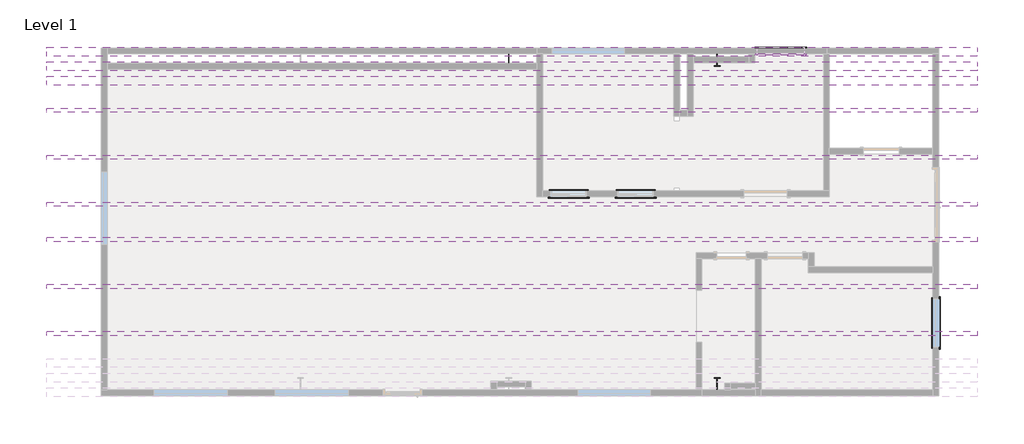
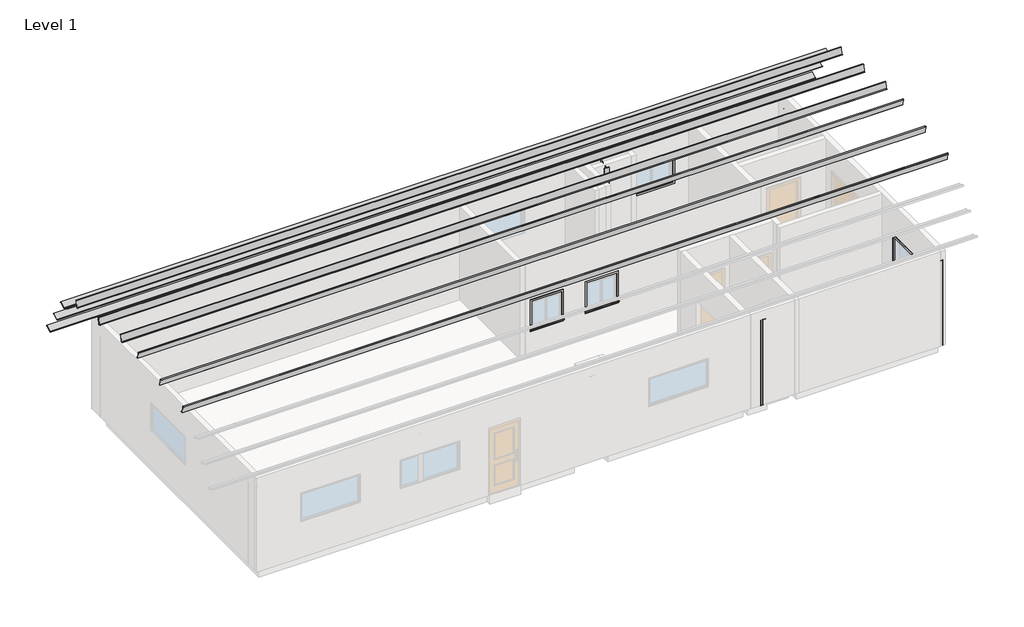
# One storey, part 3 of 3: 9 beams, 8 proxies, 5 columns.
"""IFC4 building model written with IfcOpenShell, lengths in millimetres."""

import ifcopenshell
import ifcopenshell.guid

model = None  # the IFC model being written
_history = None  # IfcOwnerHistory: only IFC2X3 demands one
_inside = {}  # id of a spatial element -> (the spatial element, [elements in it])
_under = {}  # id of a project, library or spatial element -> (it, [spatial elements below it])
_declared = {}  # id of a project -> (the project, [libraries it declares])
_typed = {}  # id of a type object -> (the type object, [elements of that type])
_made_of = {}  # id of a material, layer set ... -> (it, [elements and type objects made of it])


def new_model(schema):
    """Start an empty IFC model of exactly this schema.

    Asked for "IFC4X3", IfcOpenShell would pick the latest addendum, in which some entities
    have other attributes; the version numbers below select the first issue.
    IFC2X3 requires an IfcOwnerHistory on every rooted entity: one is made here for all.
    """
    global model, _history
    if schema == "IFC4X3":
        model = ifcopenshell.file(schema_version=(4, 3, 0, 0))
    else:
        model = ifcopenshell.file(schema=schema)
    _inside.clear()
    _under.clear()
    _declared.clear()
    _typed.clear()
    _made_of.clear()
    _history = None
    if model.schema == "IFC2X3":
        org = make("IfcOrganization", Name="unknown")
        user = make(
            "IfcPersonAndOrganization",
            ThePerson=make("IfcPerson", FamilyName="unknown"),
            TheOrganization=org,
        )
        app = make(
            "IfcApplication",
            ApplicationDeveloper=org,
            Version="unknown",
            ApplicationFullName="unknown",
            ApplicationIdentifier="unknown",
        )
        _history = make(
            "IfcOwnerHistory",
            OwningUser=user,
            OwningApplication=app,
            ChangeAction="ADDED",
            CreationDate=0,
        )
    return model


def make(cls, **values):
    """One entity of the class cls with the attributes given. An attribute that is None is left unset."""
    return model.create_entity(
        cls, **{name: value for name, value in values.items() if value is not None}
    )


def rooted(cls, **values):
    """An entity with a GlobalId (a new one), such as an element, a storey or a relation."""
    return make(cls, GlobalId=ifcopenshell.guid.new(), OwnerHistory=_history, **values)


def si_unit(unit_type, name, prefix=None):
    """IfcSIUnit, for example si_unit("LENGTHUNIT", "METRE", prefix="MILLI")."""
    return make("IfcSIUnit", UnitType=unit_type, Prefix=prefix, Name=name)


def assignment(units):
    """IfcUnitAssignment: the units of a project."""
    return None if units is None else make("IfcUnitAssignment", Units=units)


def point(xyz):
    """IfcCartesianPoint."""
    return None if xyz is None else make("IfcCartesianPoint", Coordinates=xyz)


def direction(xyz):
    """IfcDirection."""
    return None if xyz is None else make("IfcDirection", DirectionRatios=xyz)


def frame(location, z_axis=None, x_axis=None):
    """IfcAxis2Placement3D, a coordinate frame: its origin and axes. An axis left out is left unset."""
    return make(
        "IfcAxis2Placement3D",
        Location=point(location),
        Axis=direction(z_axis),
        RefDirection=direction(x_axis),
    )


def origin():
    """The frame at (0, 0, 0) with its axes left unset."""
    return frame((0.0, 0.0, 0.0))


def origin_with_axes():
    """The frame at (0, 0, 0) with the z axis (0, 0, 1) and the x axis (1, 0, 0) written out."""
    return frame((0.0, 0.0, 0.0), z_axis=(0.0, 0.0, 1.0), x_axis=(1.0, 0.0, 0.0))


def place(relative_to, where):
    """IfcLocalPlacement: puts the frame where relative to a parent placement (None: the world)."""
    return make(
        "IfcLocalPlacement", PlacementRelTo=relative_to, RelativePlacement=where
    )


def context(
    kind, dimensions, precision=None, world=None, true_north=None, identifier=None
):
    """IfcGeometricRepresentationContext, for example the 3D "Model" context."""
    return make(
        "IfcGeometricRepresentationContext",
        ContextIdentifier=identifier,
        ContextType=kind,
        CoordinateSpaceDimension=dimensions,
        Precision=precision,
        WorldCoordinateSystem=world,
        TrueNorth=true_north,
    )


def project(units=None, contexts=None):
    """IfcProject with its units and contexts."""
    return rooted(
        "IfcProject",
        Name="project",
        RepresentationContexts=contexts,
        UnitsInContext=assignment(units),
    )


def spatial(cls, under=None, at=None, **own):
    """A site, building, storey or space (cls), placed at a placement, below another one or the project."""
    s = rooted(cls, ObjectPlacement=at, **own)
    if under is not None:
        _under.setdefault(under.id(), (under, []))[1].append(s)
    return s


def polyline(points):
    """IfcPolyline through the points."""
    return make("IfcPolyline", Points=[point(p) for p in points])


def circle_curve(where, radius):
    """IfcCircle in the frame where."""
    return make("IfcCircle", Position=where, Radius=radius)


def ellipse_curve(where, semi_axis1, semi_axis2):
    """IfcEllipse in the frame where."""
    return make(
        "IfcEllipse", Position=where, SemiAxis1=semi_axis1, SemiAxis2=semi_axis2
    )


def outline(outer, holes=None, kind="AREA"):
    """IfcArbitraryClosedProfileDef: a profile drawn as a closed curve; with holes, ...WithVoids."""
    if holes is None:
        return make("IfcArbitraryClosedProfileDef", ProfileType=kind, OuterCurve=outer)
    return make(
        "IfcArbitraryProfileDefWithVoids",
        ProfileType=kind,
        OuterCurve=outer,
        InnerCurves=holes,
    )


def extrude(swept, where, along, depth):
    """IfcExtrudedAreaSolid: the profile swept, set in the frame where, extruded along a direction by depth."""
    return make(
        "IfcExtrudedAreaSolid",
        SweptArea=swept,
        Position=where,
        ExtrudedDirection=direction(along),
        Depth=depth,
    )


def shape(context_of_items, identifier, shape_type, items):
    """IfcShapeRepresentation: the items that make up one representation, for example the "Body"."""
    return make(
        "IfcShapeRepresentation",
        ContextOfItems=context_of_items,
        RepresentationIdentifier=identifier,
        RepresentationType=shape_type,
        Items=items,
    )


def source(mapping_origin, context_of_items, identifier, shape_type, items):
    """IfcRepresentationMap: a shape defined once, which mapped items show again and again."""
    return make(
        "IfcRepresentationMap",
        MappingOrigin=mapping_origin,
        MappedRepresentation=shape(context_of_items, identifier, shape_type, items),
    )


def transform(
    local_origin,
    x_axis=None,
    y_axis=None,
    z_axis=None,
    scale=None,
    scale2=None,
    scale3=None,
    uniform=True,
):
    """IfcCartesianTransformationOperator3D, or its non-uniform kind. x_axis, y_axis, z_axis: its Axis1, 2, 3."""
    if uniform:
        return make(
            "IfcCartesianTransformationOperator3D",
            Axis1=direction(x_axis),
            Axis2=direction(y_axis),
            LocalOrigin=point(local_origin),
            Scale=scale,
            Axis3=direction(z_axis),
        )
    return make(
        "IfcCartesianTransformationOperator3DnonUniform",
        Axis1=direction(x_axis),
        Axis2=direction(y_axis),
        LocalOrigin=point(local_origin),
        Scale=scale,
        Axis3=direction(z_axis),
        Scale2=scale2,
        Scale3=scale3,
    )


def mapped(mapping_source, mapping_target):
    """IfcMappedItem: shows the shape of a source again, moved by a transform."""
    return make(
        "IfcMappedItem", MappingSource=mapping_source, MappingTarget=mapping_target
    )


def made_of(thing, what):
    """Note that an element or type object is made of a material, layer set ...; save() writes the relation."""
    if what is not None:
        _made_of.setdefault(what.id(), (what, []))[1].append(thing)
    return thing


def element(
    cls,
    number,
    at=None,
    inside=None,
    cuts=None,
    type_object=None,
    material=None,
    context=None,
    identifier="Body",
    shape_type=None,
    held_by="IfcProductDefinitionShape",
    body=None,
    shapes=None,
    **own,
):
    """One element of the class cls, such as IfcWall. Its Tag is "e" and its number.

    at: its placement. inside: the storey or other place that contains it. cuts: it is an
    opening in that element (IfcRelVoidsElement). A single representation is given by context,
    identifier, shape_type and body (its items); several are given by shapes. held_by: the class
    of the entity that holds the representations. save() writes the other relations.
    """
    e = rooted(cls, Tag="e%d" % number, ObjectPlacement=at, **own)
    if body is not None:
        shapes = [shape(context, identifier, shape_type, body)]
    if shapes is not None:
        e.Representation = make(held_by, Representations=shapes)
    if inside is not None:
        _inside.setdefault(inside.id(), (inside, []))[1].append(e)
    if cuts is not None:
        rooted(
            "IfcRelVoidsElement", RelatingBuildingElement=cuts, RelatedOpeningElement=e
        )
    if type_object is not None:
        _typed.setdefault(type_object.id(), (type_object, []))[1].append(e)
    return made_of(e, material)


def aggregate(whole, parts):
    """IfcRelAggregates: a whole, such as a stair, and the parts it consists of."""
    return rooted("IfcRelAggregates", RelatingObject=whole, RelatedObjects=parts)


def save(model, path):
    """Write the relations noted so far, then the file.

    IfcRelAggregates (storeys below a building ...), IfcRelContainedInSpatialStructure (elements
    in a storey), IfcRelDefinesByType, IfcRelAssociatesMaterial and IfcRelDeclares: one each for
    every whole, place, type object, material and project.
    """
    for whole, parts in _under.values():
        aggregate(whole, parts)
    for where, things in _inside.values():
        rooted(
            "IfcRelContainedInSpatialStructure",
            RelatedElements=things,
            RelatingStructure=where,
        )
    for kind, things in _typed.values():
        rooted("IfcRelDefinesByType", RelatedObjects=things, RelatingType=kind)
    for what, things in _made_of.values():
        rooted("IfcRelAssociatesMaterial", RelatedObjects=things, RelatingMaterial=what)
    for by, libraries in _declared.values():
        rooted("IfcRelDeclares", RelatingContext=by, RelatedDefinitions=libraries)
    model.write(path)


def plane_surface(at):
    """IfcPlane: the flat surface through the origin of the frame at, square to its z axis."""
    return make("IfcPlane", Position=at)


def revolved_surface(curve, axis_point, axis_direction):
    """IfcSurfaceOfRevolution: the curve turned about the line through axis_point along axis_direction."""
    return make(
        "IfcSurfaceOfRevolution",
        SweptCurve=make("IfcArbitraryOpenProfileDef", ProfileType="CURVE", Curve=curve),
        AxisPosition=make("IfcAxis1Placement", Location=point(axis_point), Axis=direction(axis_direction)),
    )


def advanced_brep(points, edges, surfaces, faces):
    """IfcAdvancedBrep: a solid bounded by faces that lie on surfaces and meet in shared edges.

    An edge is (start, end): straight between two places in points (the first is 0);
    or (start, end, curve); or (start, end, curve, False) where it runs against its curve.
    A face is (place in surfaces, loops), or (place, loops, False) where it looks against
    its surface's normal. A loop lists edges by number (the first is 1), with a minus sign
    where the edge is run from its end to its start. The first loop is the outer one.
    """
    corners = [point(p) for p in points]
    vertices = [make("IfcVertexPoint", VertexGeometry=c) for c in corners]
    made = []
    for start, end, *more in edges:
        made.append(
            make(
                "IfcEdgeCurve",
                EdgeStart=vertices[start],
                EdgeEnd=vertices[end],
                EdgeGeometry=more[0] if more else make("IfcPolyline", Points=[corners[start], corners[end]]),
                SameSense=more[1] if len(more) > 1 else True,
            )
        )
    hull = []
    for where, loops, *sense in faces:
        bounds = []
        for j, loop in enumerate(loops):
            ring = [make("IfcOrientedEdge", EdgeElement=made[abs(k) - 1], Orientation=k > 0) for k in loop]
            bounds.append(
                make(
                    "IfcFaceOuterBound" if j == 0 else "IfcFaceBound",
                    Bound=make("IfcEdgeLoop", EdgeList=ring),
                    Orientation=True,
                )
            )
        hull.append(make("IfcAdvancedFace", Bounds=bounds, FaceSurface=surfaces[where], SameSense=sense[0] if sense else True))
    return make("IfcAdvancedBrep", Outer=make("IfcClosedShell", CfsFaces=hull))


def z_shapes_z_3x8_0ff4bf34(model_context):
    return source(origin(), model_context, "Body", "SweptSolid", [
        extrude(outline(polyline([(-57.2805719, 101.596825), (-57.2805719, 111.248825), (-19.1805719, 111.248825), (-19.1805719, -101.603175), (18.9194281, -101.603175), (18.9194281, -107.953175), (-27.1991352, -107.953175), (-27.1991352, 101.596825), (-57.2805719, 101.596825)])), frame((-11963.4, 0.0, 0.0), z_axis=(1.0, 0.0, 0.0), x_axis=(0.0, 1.0, 0.0)), (0.0, 0.0, 1.0), 23926.8),
    ])


def trim_window_exterior_flat_with_sill_c4e67c73(model_context):
    return source(origin(), model_context, "Body", "SweptSolid", [
        extrude(outline(polyline([(666.75, -936.5823709), (666.75, -993.7323709), (-666.75, -993.7323709), (-666.75, -936.5823709), (666.75, -936.5823709)])), origin_with_axes(), (0.0, 0.0, 1.0), 19.05),
        extrude(outline(polyline([(-946.15, 38.1), (-916.8580645, 38.1), (-914.4, 19.05), (-914.4, 0.0), (-936.5823709, 0.0), (-936.5823709, 19.05), (-946.15, 19.05), (-946.15, 38.1)])), frame((-679.45, 0.0, 0.0), z_axis=(1.0, 0.0, 0.0), x_axis=(0.0, 1.0, 0.0)), (0.0, 0.0, 1.0), 1358.9),
        extrude(outline(polyline([(-666.75, 57.15), (666.75, 57.15), (666.75, -914.4), (609.6, -914.4), (609.6, 0.0), (-609.6, 0.0), (-609.6, -914.4), (-666.75, -914.4), (-666.75, 57.15)])), origin_with_axes(), (0.0, 0.0, 1.0), 19.05),
    ])


def trim_window_exterior_flat_with_sill_84e24481(model_context):
    return source(origin(), model_context, "Body", "SweptSolid", [
        extrude(outline(polyline([(514.35, -936.5823709), (514.35, -993.7323709), (-514.35, -993.7323709), (-514.35, -936.5823709), (514.35, -936.5823709)])), origin_with_axes(), (0.0, 0.0, 1.0), 19.05),
        extrude(outline(polyline([(-946.15, 38.1), (-916.8580645, 38.1), (-914.4, 19.05), (-914.4, 0.0), (-936.5823709, 0.0), (-936.5823709, 19.05), (-946.15, 19.05), (-946.15, 38.1)])), frame((-527.05, 0.0, 0.0), z_axis=(1.0, 0.0, 0.0), x_axis=(0.0, 1.0, 0.0)), (0.0, 0.0, 1.0), 1054.1),
        extrude(outline(polyline([(-514.35, 57.15), (514.35, 57.15), (514.35, -914.4), (457.2, -914.4), (457.2, 0.0), (-457.2, 0.0), (-457.2, -914.4), (-514.35, -914.4), (-514.35, 57.15)])), origin_with_axes(), (0.0, 0.0, 1.0), 19.05),
    ])


def trim_window_interior_flat_picture_frame_cf1733af(model_context):
    return source(origin(), model_context, "Body", "SweptSolid", [
        extrude(outline(polyline([(654.05, 44.45), (654.05, -958.85), (-654.05, -958.85), (-654.05, 44.45), (654.05, 44.45)]), holes=[polyline([(596.9, -12.7), (-596.9, -12.7), (-596.9, -901.7), (596.9, -901.7), (596.9, -12.7)])]), origin_with_axes(), (0.0, 0.0, 1.0), 31.75),
    ])


def trim_window_interior_flat_picture_frame_28d4e5dc(model_context):
    return source(origin(), model_context, "Body", "SweptSolid", [
        extrude(outline(polyline([(501.65, 44.45), (501.65, -958.85), (-501.65, -958.85), (-501.65, 44.45), (501.65, 44.45)]), holes=[polyline([(444.5, -12.7), (-444.5, -12.7), (-444.5, -901.7), (444.5, -901.7), (444.5, -12.7)])]), origin_with_axes(), (0.0, 0.0, 1.0), 31.75),
    ])


model = new_model("IFC4")

# Units and contexts
model_context = context("Model", 3, world=origin())
ifc_project = project(units=[si_unit("LENGTHUNIT", "METRE", prefix="MILLI")], contexts=[model_context])

# Site, building, storey
site = spatial("IfcSite", under=ifc_project)
building = spatial("IfcBuilding", under=site)
storey = spatial("IfcBuildingStorey", under=building, Name="Level 1", Elevation=0.0)

# Beams
placement = place(None, origin())
z_shapes_z_3x8_shape = z_shapes_z_3x8_0ff4bf34(model_context)
element("IfcBeam", 1, ObjectType="Z Shapes : Z 3X8", at=placement, inside=storey, context=model_context, shape_type="MappedRepresentation", body=[
    mapped(z_shapes_z_3x8_shape, transform((18060.1870052, 9961.4548323, 4912.1209483), x_axis=(-1.0, 0.0, 0.0), y_axis=(0.0, -0.9907950027882196, 0.13537083308413195), z_axis=(0.0, 0.13537083308413195, 0.9907950027882196))),
])
element("IfcBeam", 2, ObjectType="Z Shapes : Z 3X8", at=placement, inside=storey, context=model_context, shape_type="MappedRepresentation", body=[
    mapped(z_shapes_z_3x8_shape, transform((18060.1870052, 8753.4775649, 5077.165068), x_axis=(-1.0, 0.0, 0.0), y_axis=(0.0, -0.9907950027882196, 0.13537083308413195), z_axis=(0.0, 0.13537083308413195, 0.9907950027882196))),
])
element("IfcBeam", 3, ObjectType="Z Shapes : Z 3X8", at=placement, inside=storey, context=model_context, shape_type="MappedRepresentation", body=[
    mapped(z_shapes_z_3x8_shape, transform((18060.1870052, 7545.5002975, 5242.2091877), x_axis=(-1.0, 0.0, 0.0), y_axis=(0.0, -0.9907950027882196, 0.13537083308413195), z_axis=(0.0, 0.13537083308413195, 0.9907950027882196))),
])
element("IfcBeam", 4, ObjectType="Z Shapes : Z 3X8", at=placement, inside=storey, context=model_context, shape_type="MappedRepresentation", body=[
    mapped(z_shapes_z_3x8_shape, transform((18060.1870052, 6681.0227757, 5242.2091877), x_axis=(1.0, 0.0, 0.0), y_axis=(0.0, 0.9907950027882196, 0.13537083308413195), z_axis=(0.0, -0.13537083308413195, 0.9907950027882196))),
])
element("IfcBeam", 5, ObjectType="Z Shapes : Z 3X8", at=placement, inside=storey, context=model_context, shape_type="MappedRepresentation", body=[
    mapped(z_shapes_z_3x8_shape, transform((18060.1870052, 5473.0455083, 5077.165068), x_axis=(1.0, 0.0, 0.0), y_axis=(0.0, 0.9907950027882196, 0.13537083308413195), z_axis=(0.0, -0.13537083308413195, 0.9907950027882196))),
])
element("IfcBeam", 6, ObjectType="Z Shapes : Z 3X8", at=placement, inside=storey, context=model_context, shape_type="MappedRepresentation", body=[
    mapped(z_shapes_z_3x8_shape, transform((18060.1870052, 4265.0682409, 4912.1209483), x_axis=(1.0, 0.0, 0.0), y_axis=(0.0, 0.9907950027882196, 0.13537083308413195), z_axis=(0.0, -0.13537083308413195, 0.9907950027882196))),
])
element("IfcBeam", 7, ObjectType="Z Shapes : Z 3X8", at=placement, inside=storey, context=model_context, shape_type="MappedRepresentation", body=[
    mapped(z_shapes_z_3x8_shape, transform((18060.1870052, 10729.7081219, 4436.794501), x_axis=(-1.0, 0.0, 0.0), y_axis=(0.0, -0.5198738321222813, 0.8542430559708952), z_axis=(0.0, 0.8542430559708952, 0.5198738321222813))),
])
element("IfcBeam", 8, ObjectType="Z Shapes : Z 3X8", at=placement, inside=storey, context=model_context, shape_type="MappedRepresentation", body=[
    mapped(z_shapes_z_3x8_shape, transform((18060.1870052, 11104.2691119, 3821.3256987), x_axis=(-1.0, 0.0, 0.0), y_axis=(0.0, -0.5198738321222813, 0.8542430559708952), z_axis=(0.0, 0.8542430559708952, 0.5198738321222813))),
])
element("IfcBeam", 9, ObjectType="Z Shapes : Z 3X8", at=placement, inside=storey, context=model_context, shape_type="MappedRepresentation", body=[
    mapped(z_shapes_z_3x8_shape, transform((18060.1870052, 11478.830102, 3205.8568965), x_axis=(-1.0, 0.0, 0.0), y_axis=(0.0, -0.5198738321222813, 0.8542430559708952), z_axis=(0.0, 0.8542430559708952, 0.5198738321222813))),
])

# Proxies
trim_window_exterior_flat_with_sill_shape = trim_window_exterior_flat_with_sill_c4e67c73(model_context)
element("IfcBuildingElementProxy", 10, Name="Trim-Window-Exterior-Flat : with Sill", ObjectType="Trim-Window-Exterior-Flat : with Sill", at=placement, inside=storey, context=model_context, shape_type="MappedRepresentation", body=[
    mapped(trim_window_exterior_flat_with_sill_shape, transform((24967.1591867, 11583.6615366, 2166.9735008), x_axis=(-1.0, 0.0, 0.0), y_axis=(0.0, 0.0, 1.0), z_axis=(0.0, 1.0, 0.0))),
])
element("IfcBuildingElementProxy", 11, Name="Trim-Window-Exterior-Flat : with Sill", ObjectType="Trim-Window-Exterior-Flat : with Sill", at=placement, inside=storey, context=model_context, shape_type="MappedRepresentation", body=[
    mapped(trim_window_exterior_flat_with_sill_shape, transform((29032.9870052, 4516.1115366, 2108.2), x_axis=(0.0, 1.0, 0.0), y_axis=(0.0, 0.0, 1.0), z_axis=(1.0, 0.0, 0.0))),
])
trim_window_exterior_flat_with_sill_2_shape = trim_window_exterior_flat_with_sill_84e24481(model_context)
element("IfcBuildingElementProxy", 12, Name="Trim-Window-Exterior-Flat : with Sill", ObjectType="Trim-Window-Exterior-Flat : with Sill", at=placement, inside=storey, context=model_context, shape_type="MappedRepresentation", body=[
    mapped(trim_window_exterior_flat_with_sill_2_shape, transform((19514.3370052, 7760.9615366, 1828.8), x_axis=(1.0, 0.0, 0.0), y_axis=(0.0, 0.0, 1.0), z_axis=(0.0, -1.0, 0.0))),
])
element("IfcBuildingElementProxy", 13, Name="Trim-Window-Exterior-Flat : with Sill", ObjectType="Trim-Window-Exterior-Flat : with Sill", at=placement, inside=storey, context=model_context, shape_type="MappedRepresentation", body=[
    mapped(trim_window_exterior_flat_with_sill_2_shape, transform((21235.1870052, 7760.9615366, 1828.8), x_axis=(1.0, 0.0, 0.0), y_axis=(0.0, 0.0, 1.0), z_axis=(0.0, -1.0, 0.0))),
])
trim_window_interior_flat_picture_frame_shape = trim_window_interior_flat_picture_frame_cf1733af(model_context)
element("IfcBuildingElementProxy", 14, Name="Trim-Window-Interior-Flat : Picture Frame", ObjectType="Trim-Window-Interior-Flat : Picture Frame", at=placement, inside=storey, context=model_context, shape_type="MappedRepresentation", body=[
    mapped(trim_window_interior_flat_picture_frame_shape, transform((24967.1591867, 11431.2615366, 2166.9735008), x_axis=(1.0, 0.0, 0.0), y_axis=(0.0, 0.0, 1.0), z_axis=(0.0, -1.0, 0.0))),
])
element("IfcBuildingElementProxy", 15, Name="Trim-Window-Interior-Flat : Picture Frame", ObjectType="Trim-Window-Interior-Flat : Picture Frame", at=placement, inside=storey, context=model_context, shape_type="MappedRepresentation", body=[
    mapped(trim_window_interior_flat_picture_frame_shape, transform((28880.5870052, 4516.1115366, 2108.2), x_axis=(0.0, -1.0, 0.0), y_axis=(0.0, 0.0, 1.0), z_axis=(-1.0, 0.0, 0.0))),
])
trim_window_interior_flat_picture_frame_2_shape = trim_window_interior_flat_picture_frame_28d4e5dc(model_context)
element("IfcBuildingElementProxy", 16, Name="Trim-Window-Interior-Flat : Picture Frame", ObjectType="Trim-Window-Interior-Flat : Picture Frame", at=placement, inside=storey, context=model_context, shape_type="MappedRepresentation", body=[
    mapped(trim_window_interior_flat_picture_frame_2_shape, transform((19514.3370052, 7913.3615366, 1828.8), x_axis=(-1.0, 0.0, 0.0), y_axis=(0.0, 0.0, 1.0), z_axis=(0.0, 1.0, 0.0))),
])
element("IfcBuildingElementProxy", 17, Name="Trim-Window-Interior-Flat : Picture Frame", ObjectType="Trim-Window-Interior-Flat : Picture Frame", at=placement, inside=storey, context=model_context, shape_type="MappedRepresentation", body=[
    mapped(trim_window_interior_flat_picture_frame_2_shape, transform((21235.1870052, 7913.3615366, 1828.8), x_axis=(-1.0, 0.0, 0.0), y_axis=(0.0, 0.0, 1.0), z_axis=(0.0, 1.0, 0.0))),
])

# Columns
element("IfcColumn", 18, ObjectType="W-Wide Flange-Column : W6X18.5", at=placement, inside=storey, context=model_context, shape_type="AdvancedBrep", body=[
    advanced_brep(
    [(29032.9870052, 11583.6615366, 0.0), (29032.9870052, 11573.3745366, 0.0), (28972.0270052, 11573.3745366, 0.0), (28960.0890052, 11561.4365366, 0.0), (28960.0890052, 11135.9865366, 0.0), (28972.0270052, 11124.0485366, 0.0), (29032.9870052, 11124.0485366, 0.0), (29032.9870052, 11113.7615366, 0.0), (28880.5870052, 11113.7615366, 0.0), (28880.5870052, 11124.0485366, 0.0), (28941.5470052, 11124.0485366, 0.0), (28953.4850052, 11135.9865366, 0.0), (28953.4850052, 11561.4365366, 0.0), (28941.5470052, 11573.3745366, 0.0), (28880.5870052, 11573.3745366, 0.0), (28880.5870052, 11583.6615366, 0.0), (29032.9870052, 11583.6615366, 2825.947988), (29032.9870052, 11573.3745366, 2823.0639572), (28972.0270052, 11573.3745366, 2823.0639572), (28960.0890052, 11561.4365366, 2819.7170571), (28960.0890052, 11135.9865366, 2700.4392375), (28972.0270052, 11124.0485366, 2697.0923375), (29032.9870052, 11124.0485366, 2697.0923375), (29032.9870052, 11113.7615366, 2694.2083066), (28880.5870052, 11113.7615366, 2694.2083066), (28880.5870052, 11124.0485366, 2697.0923375), (28941.5470052, 11124.0485366, 2697.0923375), (28953.4850052, 11135.9865366, 2700.4392375), (28953.4850052, 11561.4365366, 2819.7170571), (28941.5470052, 11573.3745366, 2823.0639572), (28880.5870052, 11573.3745366, 2823.0639572), (28880.5870052, 11583.6615366, 2825.947988)],
    [
        (0, 1),
        (1, 2),
        (2, 3, circle_curve(frame((28972.0270052, 11561.4365366, 0.0), z_axis=(0.0, 0.0, 1.0), x_axis=(1.0, 0.0, 0.0)), 11.938)),
        (3, 4),
        (4, 5, circle_curve(frame((28972.0270052, 11135.9865366, 0.0), z_axis=(0.0, 0.0, 1.0), x_axis=(1.0, 0.0, 0.0)), 11.938)),
        (5, 6),
        (6, 7),
        (7, 8),
        (8, 9),
        (9, 10),
        (10, 11, circle_curve(frame((28941.5470052, 11135.9865366, 0.0), z_axis=(0.0, 0.0, 1.0), x_axis=(1.0, 0.0, 0.0)), 11.938)),
        (11, 12),
        (12, 13, circle_curve(frame((28941.5470052, 11561.4365366, 0.0), z_axis=(0.0, 0.0, 1.0), x_axis=(1.0, 0.0, 0.0)), 11.938)),
        (13, 14),
        (14, 15),
        (15, 0),
        (0, 16),
        (16, 17),
        (17, 1),
        (17, 18),
        (18, 2),
        (18, 19, ellipse_curve(frame((28972.0270052, 11561.4365366, 2819.7170571), z_axis=(0.0, -0.2699485280248176, 0.9628747541696346), x_axis=(0.0, -0.9628747541696346, -0.2699485280248172)), 12.3982895, 11.938)),
        (19, 3),
        (19, 20),
        (20, 4),
        (20, 21, ellipse_curve(frame((28972.0270052, 11135.9865366, 2700.4392375), z_axis=(0.0, -0.2699485280248176, 0.9628747541696346), x_axis=(0.0, -0.9628747541696346, -0.2699485280248172)), 12.3982895, 11.938)),
        (21, 5),
        (21, 22),
        (22, 6),
        (22, 23),
        (23, 7),
        (23, 24),
        (24, 8),
        (24, 25),
        (25, 9),
        (25, 26),
        (26, 10),
        (26, 27, ellipse_curve(frame((28941.5470052, 11135.9865366, 2700.4392375), z_axis=(0.0, -0.2699485280248176, 0.9628747541696346), x_axis=(0.0, -0.9628747541696346, -0.2699485280248172)), 12.3982895, 11.938)),
        (27, 11),
        (27, 28),
        (28, 12),
        (28, 29, ellipse_curve(frame((28941.5470052, 11561.4365366, 2819.7170571), z_axis=(0.0, -0.2699485280248176, 0.9628747541696346), x_axis=(0.0, -0.9628747541696346, -0.2699485280248172)), 12.3982895, 11.938)),
        (29, 13),
        (29, 30),
        (30, 14),
        (30, 31),
        (31, 15),
        (31, 16),
    ],
    [
        plane_surface(frame((28880.5870052, 11583.6615366, 0.0), z_axis=(0.0, 0.0, -1.0), x_axis=(1.0, 0.0, 0.0))),
        plane_surface(frame((29032.9870052, 11573.3745366, 2832.1), z_axis=(1.0, 0.0, 0.0), x_axis=(0.0, 0.0, -1.0))),
        plane_surface(frame((28972.0270052, 11573.3745366, 2832.1), z_axis=(0.0, -1.0, 0.0), x_axis=(0.0, 0.0, -1.0))),
        revolved_surface(polyline([(28983.9650052, 11561.4365366, 0.0), (28983.9650052, 11561.4365366, 2823.0639572)]), (28972.0270052, 11561.4365366, 0.0), (0.0, 0.0, -1.0)),
        plane_surface(frame((28960.0890052, 11135.9865366, 2832.1), z_axis=(1.0, 0.0, 0.0), x_axis=(0.0, 0.0, -1.0))),
        revolved_surface(polyline([(28983.9650052, 11135.9865366, 0.0), (28983.9650052, 11135.9865366, 2703.786137500551)]), (28972.0270052, 11135.9865366, 0.0), (0.0, 0.0, -1.0)),
        plane_surface(frame((29032.9870052, 11124.0485366, 2832.1), z_axis=(0.0, 1.0, 0.0), x_axis=(0.0, 0.0, -1.0))),
        plane_surface(frame((29032.9870052, 11113.7615366, 2832.1), z_axis=(1.0, 0.0, 0.0), x_axis=(0.0, 0.0, -1.0))),
        plane_surface(frame((28880.5870052, 11113.7615366, 2832.1), z_axis=(0.0, -1.0, 0.0), x_axis=(0.0, 0.0, -1.0))),
        plane_surface(frame((28880.5870052, 11124.0485366, 2832.1), z_axis=(-1.0, 0.0, 0.0), x_axis=(0.0, 0.0, -1.0))),
        plane_surface(frame((28941.5470052, 11124.0485366, 2832.1), z_axis=(0.0, 1.0, 0.0), x_axis=(0.0, 0.0, -1.0))),
        revolved_surface(polyline([(28953.485005199997, 11135.9865366, 0.0), (28953.485005199997, 11135.9865366, 2703.786137500551)]), (28941.5470052, 11135.9865366, 0.0), (0.0, 0.0, -1.0)),
        plane_surface(frame((28953.4850052, 11561.4365366, 2832.1), z_axis=(-1.0, 0.0, 0.0), x_axis=(0.0, 0.0, -1.0))),
        revolved_surface(polyline([(28953.485005199997, 11561.4365366, 0.0), (28953.485005199997, 11561.4365366, 2823.0639572)]), (28941.5470052, 11561.4365366, 0.0), (0.0, 0.0, -1.0)),
        plane_surface(frame((28880.5870052, 11573.3745366, 2832.1), z_axis=(0.0, -1.0, 0.0), x_axis=(0.0, 0.0, -1.0))),
        plane_surface(frame((28880.5870052, 11583.6615366, 2832.1), z_axis=(-1.0, 0.0, 0.0), x_axis=(0.0, 0.0, -1.0))),
        plane_surface(frame((29032.9870052, 11583.6615366, 2832.1), z_axis=(0.0, 1.0, 0.0), x_axis=(0.0, 0.0, -1.0))),
        plane_surface(frame((26124.6870052, 11722.0217176, 2864.7382118), z_axis=(0.0, -0.2699485280248176, 0.9628747541696346), x_axis=(1.0, 0.0, 0.0))),
    ],
    [
        (0, [[1, 2, 3, 4, 5, 6, 7, 8, 9, 10, 11, 12, 13, 14, 15, 16]]),
        (1, [[-1, 17, 18, 19]]),
        (2, [[-2, -19, 20, 21]]),
        (3, [[-3, -21, 22, 23]]),
        (4, [[-4, -23, 24, 25]]),
        (5, [[-5, -25, 26, 27]]),
        (6, [[-6, -27, 28, 29]]),
        (7, [[-7, -29, 30, 31]]),
        (8, [[-8, -31, 32, 33]]),
        (9, [[-9, -33, 34, 35]]),
        (10, [[-10, -35, 36, 37]]),
        (11, [[-11, -37, 38, 39]]),
        (12, [[-12, -39, 40, 41]]),
        (13, [[-13, -41, 42, 43]]),
        (14, [[-14, -43, 44, 45]]),
        (15, [[-15, -45, 46, 47]]),
        (16, [[-16, -47, 48, -17]]),
        (17, [[-18, -48, -46, -44, -42, -40, -38, -36, -34, -32, -30, -28, -26, -24, -22, -20]]),
    ],
),
])
element("IfcColumn", 19, ObjectType="W-Wide Flange-Column : W6X18.5", at=placement, inside=storey, context=model_context, shape_type="AdvancedBrep", body=[
    advanced_brep(
    [(28880.5870052, 2642.8615366, 0.0), (28880.5870052, 2653.1485366, 0.0), (28941.5470052, 2653.1485366, 0.0), (28953.4850052, 2665.0865366, 0.0), (28953.4850052, 3090.5365366, 0.0), (28941.5470052, 3102.4745366, 0.0), (28880.5870052, 3102.4745366, 0.0), (28880.5870052, 3112.7615366, 0.0), (29032.9870052, 3112.7615366, 0.0), (29032.9870052, 3102.4745366, 0.0), (28972.0270052, 3102.4745366, 0.0), (28960.0890052, 3090.5365366, 0.0), (28960.0890052, 2665.0865366, 0.0), (28972.0270052, 2653.1485366, 0.0), (29032.9870052, 2653.1485366, 0.0), (29032.9870052, 2642.8615366, 0.0), (28880.5870052, 2642.8615366, 2825.947988), (28880.5870052, 2653.1485366, 2823.0639572), (28941.5470052, 2653.1485366, 2823.0639572), (28953.4850052, 2665.0865366, 2819.7170571), (28953.4850052, 3090.5365366, 2700.4392375), (28941.5470052, 3102.4745366, 2697.0923375), (28880.5870052, 3102.4745366, 2697.0923375), (28880.5870052, 3112.7615366, 2694.2083066), (29032.9870052, 3112.7615366, 2694.2083066), (29032.9870052, 3102.4745366, 2697.0923375), (28972.0270052, 3102.4745366, 2697.0923375), (28960.0890052, 3090.5365366, 2700.4392375), (28960.0890052, 2665.0865366, 2819.7170571), (28972.0270052, 2653.1485366, 2823.0639572), (29032.9870052, 2653.1485366, 2823.0639572), (29032.9870052, 2642.8615366, 2825.947988)],
    [
        (0, 1),
        (1, 2),
        (2, 3, circle_curve(frame((28941.5470052, 2665.0865366, 0.0), z_axis=(0.0, 0.0, 1.0), x_axis=(-1.0, 0.0, 0.0)), 11.938)),
        (3, 4),
        (4, 5, circle_curve(frame((28941.5470052, 3090.5365366, 0.0), z_axis=(0.0, 0.0, 1.0), x_axis=(-1.0, 0.0, 0.0)), 11.938)),
        (5, 6),
        (6, 7),
        (7, 8),
        (8, 9),
        (9, 10),
        (10, 11, circle_curve(frame((28972.0270052, 3090.5365366, 0.0), z_axis=(0.0, 0.0, 1.0), x_axis=(-1.0, 0.0, 0.0)), 11.938)),
        (11, 12),
        (12, 13, circle_curve(frame((28972.0270052, 2665.0865366, 0.0), z_axis=(0.0, 0.0, 1.0), x_axis=(-1.0, 0.0, 0.0)), 11.938)),
        (13, 14),
        (14, 15),
        (15, 0),
        (0, 16),
        (16, 17),
        (17, 1),
        (17, 18),
        (18, 2),
        (18, 19, ellipse_curve(frame((28941.5470052, 2665.0865366, 2819.7170571), z_axis=(0.0, 0.2699485280248176, 0.9628747541696346), x_axis=(0.0, 0.9628747541696346, -0.2699485280248172)), 12.3982895, 11.938)),
        (19, 3),
        (19, 20),
        (20, 4),
        (20, 21, ellipse_curve(frame((28941.5470052, 3090.5365366, 2700.4392375), z_axis=(0.0, 0.2699485280248176, 0.9628747541696346), x_axis=(0.0, 0.9628747541696346, -0.2699485280248172)), 12.3982895, 11.938)),
        (21, 5),
        (21, 22),
        (22, 6),
        (22, 23),
        (23, 7),
        (23, 24),
        (24, 8),
        (24, 25),
        (25, 9),
        (25, 26),
        (26, 10),
        (26, 27, ellipse_curve(frame((28972.0270052, 3090.5365366, 2700.4392375), z_axis=(0.0, 0.2699485280248176, 0.9628747541696346), x_axis=(0.0, 0.9628747541696346, -0.2699485280248172)), 12.3982895, 11.938)),
        (27, 11),
        (27, 28),
        (28, 12),
        (28, 29, ellipse_curve(frame((28972.0270052, 2665.0865366, 2819.7170571), z_axis=(0.0, 0.2699485280248176, 0.9628747541696346), x_axis=(0.0, 0.9628747541696346, -0.2699485280248172)), 12.3982895, 11.938)),
        (29, 13),
        (29, 30),
        (30, 14),
        (30, 31),
        (31, 15),
        (31, 16),
    ],
    [
        plane_surface(frame((29032.9870052, 2642.8615366, 0.0), z_axis=(0.0, 0.0, -1.0), x_axis=(-1.0, 0.0, 0.0))),
        plane_surface(frame((28880.5870052, 2653.1485366, 2832.1), z_axis=(-1.0, 0.0, 0.0), x_axis=(0.0, 0.0, -1.0))),
        plane_surface(frame((28941.5470052, 2653.1485366, 2832.1), z_axis=(0.0, 1.0, 0.0), x_axis=(0.0, 0.0, -1.0))),
        revolved_surface(polyline([(28929.6090052, 2665.0865366, 0.0), (28929.6090052, 2665.0865366, 2823.0639572)]), (28941.5470052, 2665.0865366, 0.0), (0.0, 0.0, -1.0)),
        plane_surface(frame((28953.4850052, 3090.5365366, 2832.1), z_axis=(-1.0, 0.0, 0.0), x_axis=(0.0, 0.0, -1.0))),
        revolved_surface(polyline([(28929.6090052, 3090.5365366, 0.0), (28929.6090052, 3090.5365366, 2703.786137500551)]), (28941.5470052, 3090.5365366, 0.0), (0.0, 0.0, -1.0)),
        plane_surface(frame((28880.5870052, 3102.4745366, 2832.1), z_axis=(0.0, -1.0, 0.0), x_axis=(0.0, 0.0, -1.0))),
        plane_surface(frame((28880.5870052, 3112.7615366, 2832.1), z_axis=(-1.0, 0.0, 0.0), x_axis=(0.0, 0.0, -1.0))),
        plane_surface(frame((29032.9870052, 3112.7615366, 2832.1), z_axis=(0.0, 1.0, 0.0), x_axis=(0.0, 0.0, -1.0))),
        plane_surface(frame((29032.9870052, 3102.4745366, 2832.1), z_axis=(1.0, 0.0, 0.0), x_axis=(0.0, 0.0, -1.0))),
        plane_surface(frame((28972.0270052, 3102.4745366, 2832.1), z_axis=(0.0, -1.0, 0.0), x_axis=(0.0, 0.0, -1.0))),
        revolved_surface(polyline([(28960.089005200003, 3090.5365366, 0.0), (28960.089005200003, 3090.5365366, 2703.786137500551)]), (28972.0270052, 3090.5365366, 0.0), (0.0, 0.0, -1.0)),
        plane_surface(frame((28960.0890052, 2665.0865366, 2832.1), z_axis=(1.0, 0.0, 0.0), x_axis=(0.0, 0.0, -1.0))),
        revolved_surface(polyline([(28960.089005200003, 2665.0865366, 0.0), (28960.089005200003, 2665.0865366, 2823.0639572)]), (28972.0270052, 2665.0865366, 0.0), (0.0, 0.0, -1.0)),
        plane_surface(frame((29032.9870052, 2653.1485366, 2832.1), z_axis=(0.0, 1.0, 0.0), x_axis=(0.0, 0.0, -1.0))),
        plane_surface(frame((29032.9870052, 2642.8615366, 2832.1), z_axis=(1.0, 0.0, 0.0), x_axis=(0.0, 0.0, -1.0))),
        plane_surface(frame((28880.5870052, 2642.8615366, 2832.1), z_axis=(0.0, -1.0, 0.0), x_axis=(0.0, 0.0, -1.0))),
        plane_surface(frame((31788.8870052, 2504.5013556, 2864.7382118), z_axis=(0.0, 0.2699485280248176, 0.9628747541696346), x_axis=(-1.0, 0.0, 0.0))),
    ],
    [
        (0, [[1, 2, 3, 4, 5, 6, 7, 8, 9, 10, 11, 12, 13, 14, 15, 16]]),
        (1, [[-1, 17, 18, 19]]),
        (2, [[-2, -19, 20, 21]]),
        (3, [[-3, -21, 22, 23]]),
        (4, [[-4, -23, 24, 25]]),
        (5, [[-5, -25, 26, 27]]),
        (6, [[-6, -27, 28, 29]]),
        (7, [[-7, -29, 30, 31]]),
        (8, [[-8, -31, 32, 33]]),
        (9, [[-9, -33, 34, 35]]),
        (10, [[-10, -35, 36, 37]]),
        (11, [[-11, -37, 38, 39]]),
        (12, [[-12, -39, 40, 41]]),
        (13, [[-13, -41, 42, 43]]),
        (14, [[-14, -43, 44, 45]]),
        (15, [[-15, -45, 46, 47]]),
        (16, [[-16, -47, 48, -17]]),
        (17, [[-18, -48, -46, -44, -42, -40, -38, -36, -34, -32, -30, -28, -26, -24, -22, -20]]),
    ],
),
])
element("IfcColumn", 20, ObjectType="W-Wide Flange-Column : W6X18.5", at=placement, inside=storey, context=model_context, shape_type="AdvancedBrep", body=[
    advanced_brep(
    [(23406.8870052, 11583.6615366, 0.0), (23406.8870052, 11573.3745366, 0.0), (23345.9270052, 11573.3745366, 0.0), (23333.9890052, 11561.4365366, 0.0), (23333.9890052, 11135.9865366, 0.0), (23345.9270052, 11124.0485366, 0.0), (23406.8870052, 11124.0485366, 0.0), (23406.8870052, 11113.7615366, 0.0), (23254.4870052, 11113.7615366, 0.0), (23254.4870052, 11124.0485366, 0.0), (23315.4470052, 11124.0485366, 0.0), (23327.3850052, 11135.9865366, 0.0), (23327.3850052, 11561.4365366, 0.0), (23315.4470052, 11573.3745366, 0.0), (23254.4870052, 11573.3745366, 0.0), (23254.4870052, 11583.6615366, 0.0), (23406.8870052, 11583.6615366, 2825.947988), (23406.8870052, 11573.3745366, 2823.0639572), (23345.9270052, 11573.3745366, 2823.0639572), (23333.9890052, 11561.4365366, 2819.7170571), (23333.9890052, 11135.9865366, 2700.4392375), (23345.9270052, 11124.0485366, 2697.0923375), (23406.8870052, 11124.0485366, 2697.0923375), (23406.8870052, 11113.7615366, 2694.2083066), (23254.4870052, 11113.7615366, 2694.2083066), (23254.4870052, 11124.0485366, 2697.0923375), (23315.4470052, 11124.0485366, 2697.0923375), (23327.3850052, 11135.9865366, 2700.4392375), (23327.3850052, 11561.4365366, 2819.7170571), (23315.4470052, 11573.3745366, 2823.0639572), (23254.4870052, 11573.3745366, 2823.0639572), (23254.4870052, 11583.6615366, 2825.947988)],
    [
        (0, 1),
        (1, 2),
        (2, 3, circle_curve(frame((23345.9270052, 11561.4365366, 0.0), z_axis=(0.0, 0.0, 1.0), x_axis=(1.0, 0.0, 0.0)), 11.938)),
        (3, 4),
        (4, 5, circle_curve(frame((23345.9270052, 11135.9865366, 0.0), z_axis=(0.0, 0.0, 1.0), x_axis=(1.0, 0.0, 0.0)), 11.938)),
        (5, 6),
        (6, 7),
        (7, 8),
        (8, 9),
        (9, 10),
        (10, 11, circle_curve(frame((23315.4470052, 11135.9865366, 0.0), z_axis=(0.0, 0.0, 1.0), x_axis=(1.0, 0.0, 0.0)), 11.938)),
        (11, 12),
        (12, 13, circle_curve(frame((23315.4470052, 11561.4365366, 0.0), z_axis=(0.0, 0.0, 1.0), x_axis=(1.0, 0.0, 0.0)), 11.938)),
        (13, 14),
        (14, 15),
        (15, 0),
        (0, 16),
        (16, 17),
        (17, 1),
        (17, 18),
        (18, 2),
        (18, 19, ellipse_curve(frame((23345.9270052, 11561.4365366, 2819.7170571), z_axis=(0.0, -0.26994852802481994, 0.962874754169634), x_axis=(0.0, -0.9628747541696339, -0.26994852802481983)), 12.3982895, 11.938)),
        (19, 3),
        (19, 20),
        (20, 4),
        (20, 21, ellipse_curve(frame((23345.9270052, 11135.9865366, 2700.4392375), z_axis=(0.0, -0.26994852802481994, 0.962874754169634), x_axis=(0.0, -0.9628747541696339, -0.26994852802481983)), 12.3982895, 11.938)),
        (21, 5),
        (21, 22),
        (22, 6),
        (22, 23),
        (23, 7),
        (23, 24),
        (24, 8),
        (24, 25),
        (25, 9),
        (25, 26),
        (26, 10),
        (26, 27, ellipse_curve(frame((23315.4470052, 11135.9865366, 2700.4392375), z_axis=(0.0, -0.26994852802481994, 0.962874754169634), x_axis=(0.0, -0.9628747541696339, -0.26994852802481983)), 12.3982895, 11.938)),
        (27, 11),
        (27, 28),
        (28, 12),
        (28, 29, ellipse_curve(frame((23315.4470052, 11561.4365366, 2819.7170571), z_axis=(0.0, -0.26994852802481994, 0.962874754169634), x_axis=(0.0, -0.9628747541696339, -0.26994852802481983)), 12.3982895, 11.938)),
        (29, 13),
        (29, 30),
        (30, 14),
        (30, 31),
        (31, 15),
        (31, 16),
    ],
    [
        plane_surface(frame((23254.4870052, 11583.6615366, 0.0), z_axis=(0.0, 0.0, -1.0), x_axis=(1.0, 0.0, 0.0))),
        plane_surface(frame((23406.8870052, 11573.3745366, 2832.1), z_axis=(1.0, 0.0, 0.0), x_axis=(0.0, 0.0, -1.0))),
        plane_surface(frame((23345.9270052, 11573.3745366, 2832.1), z_axis=(0.0, -1.0, 0.0), x_axis=(0.0, 0.0, -1.0))),
        revolved_surface(polyline([(23357.865005199998, 11561.4365366, 0.0), (23357.865005199998, 11561.4365366, 2823.0639572)]), (23345.9270052, 11561.4365366, 0.0), (0.0, 0.0, -1.0)),
        plane_surface(frame((23333.9890052, 11135.9865366, 2832.1), z_axis=(1.0, 0.0, 0.0), x_axis=(0.0, 0.0, -1.0))),
        revolved_surface(polyline([(23357.865005199998, 11135.9865366, 0.0), (23357.865005199998, 11135.9865366, 2703.786137500551)]), (23345.9270052, 11135.9865366, 0.0), (0.0, 0.0, -1.0)),
        plane_surface(frame((23406.8870052, 11124.0485366, 2832.1), z_axis=(0.0, 1.0, 0.0), x_axis=(0.0, 0.0, -1.0))),
        plane_surface(frame((23406.8870052, 11113.7615366, 2832.1), z_axis=(1.0, 0.0, 0.0), x_axis=(0.0, 0.0, -1.0))),
        plane_surface(frame((23254.4870052, 11113.7615366, 2832.1), z_axis=(0.0, -1.0, 0.0), x_axis=(0.0, 0.0, -1.0))),
        plane_surface(frame((23254.4870052, 11124.0485366, 2832.1), z_axis=(-1.0, 0.0, 0.0), x_axis=(0.0, 0.0, -1.0))),
        plane_surface(frame((23315.4470052, 11124.0485366, 2832.1), z_axis=(0.0, 1.0, 0.0), x_axis=(0.0, 0.0, -1.0))),
        revolved_surface(polyline([(23327.385005199998, 11135.9865366, 0.0), (23327.385005199998, 11135.9865366, 2703.786137500551)]), (23315.4470052, 11135.9865366, 0.0), (0.0, 0.0, -1.0)),
        plane_surface(frame((23327.3850052, 11561.4365366, 2832.1), z_axis=(-1.0, 0.0, 0.0), x_axis=(0.0, 0.0, -1.0))),
        revolved_surface(polyline([(23327.385005199998, 11561.4365366, 0.0), (23327.385005199998, 11561.4365366, 2823.0639572)]), (23315.4470052, 11561.4365366, 0.0), (0.0, 0.0, -1.0)),
        plane_surface(frame((23254.4870052, 11573.3745366, 2832.1), z_axis=(0.0, -1.0, 0.0), x_axis=(0.0, 0.0, -1.0))),
        plane_surface(frame((23254.4870052, 11583.6615366, 2832.1), z_axis=(-1.0, 0.0, 0.0), x_axis=(0.0, 0.0, -1.0))),
        plane_surface(frame((23406.8870052, 11583.6615366, 2832.1), z_axis=(0.0, 1.0, 0.0), x_axis=(0.0, 0.0, -1.0))),
        plane_surface(frame((20498.5870052, 11722.0217176, 2864.7382118), z_axis=(0.0, -0.26994852802481994, 0.962874754169634), x_axis=(1.0, 0.0, 0.0))),
    ],
    [
        (0, [[1, 2, 3, 4, 5, 6, 7, 8, 9, 10, 11, 12, 13, 14, 15, 16]]),
        (1, [[-1, 17, 18, 19]]),
        (2, [[-2, -19, 20, 21]]),
        (3, [[-3, -21, 22, 23]]),
        (4, [[-4, -23, 24, 25]]),
        (5, [[-5, -25, 26, 27]]),
        (6, [[-6, -27, 28, 29]]),
        (7, [[-7, -29, 30, 31]]),
        (8, [[-8, -31, 32, 33]]),
        (9, [[-9, -33, 34, 35]]),
        (10, [[-10, -35, 36, 37]]),
        (11, [[-11, -37, 38, 39]]),
        (12, [[-12, -39, 40, 41]]),
        (13, [[-13, -41, 42, 43]]),
        (14, [[-14, -43, 44, 45]]),
        (15, [[-15, -45, 46, 47]]),
        (16, [[-16, -47, 48, -17]]),
        (17, [[-18, -48, -46, -44, -42, -40, -38, -36, -34, -32, -30, -28, -26, -24, -22, -20]]),
    ],
),
])
element("IfcColumn", 21, ObjectType="W-Wide Flange-Column : W6X18.5", at=placement, inside=storey, context=model_context, shape_type="AdvancedBrep", body=[
    advanced_brep(
    [(23254.4870052, 2642.8615366, 0.0), (23254.4870052, 2653.1485366, 0.0), (23315.4470052, 2653.1485366, 0.0), (23327.3850052, 2665.0865366, 0.0), (23327.3850052, 3090.5365366, 0.0), (23315.4470052, 3102.4745366, 0.0), (23254.4870052, 3102.4745366, 0.0), (23254.4870052, 3112.7615366, 0.0), (23406.8870052, 3112.7615366, 0.0), (23406.8870052, 3102.4745366, 0.0), (23345.9270052, 3102.4745366, 0.0), (23333.9890052, 3090.5365366, 0.0), (23333.9890052, 2665.0865366, 0.0), (23345.9270052, 2653.1485366, 0.0), (23406.8870052, 2653.1485366, 0.0), (23406.8870052, 2642.8615366, 0.0), (23254.4870052, 2642.8615366, 2825.947988), (23254.4870052, 2653.1485366, 2823.0639572), (23315.4470052, 2653.1485366, 2823.0639572), (23327.3850052, 2665.0865366, 2819.7170571), (23327.3850052, 3090.5365366, 2700.4392375), (23315.4470052, 3102.4745366, 2697.0923375), (23254.4870052, 3102.4745366, 2697.0923375), (23254.4870052, 3112.7615366, 2694.2083066), (23406.8870052, 3112.7615366, 2694.2083066), (23406.8870052, 3102.4745366, 2697.0923375), (23345.9270052, 3102.4745366, 2697.0923375), (23333.9890052, 3090.5365366, 2700.4392375), (23333.9890052, 2665.0865366, 2819.7170571), (23345.9270052, 2653.1485366, 2823.0639572), (23406.8870052, 2653.1485366, 2823.0639572), (23406.8870052, 2642.8615366, 2825.947988)],
    [
        (0, 1),
        (1, 2),
        (2, 3, circle_curve(frame((23315.4470052, 2665.0865366, 0.0), z_axis=(0.0, 0.0, 1.0), x_axis=(-1.0, 0.0, 0.0)), 11.938)),
        (3, 4),
        (4, 5, circle_curve(frame((23315.4470052, 3090.5365366, 0.0), z_axis=(0.0, 0.0, 1.0), x_axis=(-1.0, 0.0, 0.0)), 11.938)),
        (5, 6),
        (6, 7),
        (7, 8),
        (8, 9),
        (9, 10),
        (10, 11, circle_curve(frame((23345.9270052, 3090.5365366, 0.0), z_axis=(0.0, 0.0, 1.0), x_axis=(-1.0, 0.0, 0.0)), 11.938)),
        (11, 12),
        (12, 13, circle_curve(frame((23345.9270052, 2665.0865366, 0.0), z_axis=(0.0, 0.0, 1.0), x_axis=(-1.0, 0.0, 0.0)), 11.938)),
        (13, 14),
        (14, 15),
        (15, 0),
        (0, 16),
        (16, 17),
        (17, 1),
        (17, 18),
        (18, 2),
        (18, 19, ellipse_curve(frame((23315.4470052, 2665.0865366, 2819.7170571), z_axis=(0.0, 0.2699485280248201, 0.962874754169634), x_axis=(0.0, 0.962874754169634, -0.26994852802481967)), 12.3982895, 11.938)),
        (19, 3),
        (19, 20),
        (20, 4),
        (20, 21, ellipse_curve(frame((23315.4470052, 3090.5365366, 2700.4392375), z_axis=(0.0, 0.2699485280248201, 0.962874754169634), x_axis=(0.0, 0.962874754169634, -0.26994852802481967)), 12.3982895, 11.938)),
        (21, 5),
        (21, 22),
        (22, 6),
        (22, 23),
        (23, 7),
        (23, 24),
        (24, 8),
        (24, 25),
        (25, 9),
        (25, 26),
        (26, 10),
        (26, 27, ellipse_curve(frame((23345.9270052, 3090.5365366, 2700.4392375), z_axis=(0.0, 0.2699485280248201, 0.962874754169634), x_axis=(0.0, 0.962874754169634, -0.26994852802481967)), 12.3982895, 11.938)),
        (27, 11),
        (27, 28),
        (28, 12),
        (28, 29, ellipse_curve(frame((23345.9270052, 2665.0865366, 2819.7170571), z_axis=(0.0, 0.2699485280248201, 0.962874754169634), x_axis=(0.0, 0.962874754169634, -0.26994852802481967)), 12.3982895, 11.938)),
        (29, 13),
        (29, 30),
        (30, 14),
        (30, 31),
        (31, 15),
        (31, 16),
    ],
    [
        plane_surface(frame((23406.8870052, 2642.8615366, 0.0), z_axis=(0.0, 0.0, -1.0), x_axis=(-1.0, 0.0, 0.0))),
        plane_surface(frame((23254.4870052, 2653.1485366, 2832.1), z_axis=(-1.0, 0.0, 0.0), x_axis=(0.0, 0.0, -1.0))),
        plane_surface(frame((23315.4470052, 2653.1485366, 2832.1), z_axis=(0.0, 1.0, 0.0), x_axis=(0.0, 0.0, -1.0))),
        revolved_surface(polyline([(23303.5090052, 2665.0865366, 0.0), (23303.5090052, 2665.0865366, 2823.0639572)]), (23315.4470052, 2665.0865366, 0.0), (0.0, 0.0, -1.0)),
        plane_surface(frame((23327.3850052, 3090.5365366, 2832.1), z_axis=(-1.0, 0.0, 0.0), x_axis=(0.0, 0.0, -1.0))),
        revolved_surface(polyline([(23303.5090052, 3090.5365366, 0.0), (23303.5090052, 3090.5365366, 2703.786137500551)]), (23315.4470052, 3090.5365366, 0.0), (0.0, 0.0, -1.0)),
        plane_surface(frame((23254.4870052, 3102.4745366, 2832.1), z_axis=(0.0, -1.0, 0.0), x_axis=(0.0, 0.0, -1.0))),
        plane_surface(frame((23254.4870052, 3112.7615366, 2832.1), z_axis=(-1.0, 0.0, 0.0), x_axis=(0.0, 0.0, -1.0))),
        plane_surface(frame((23406.8870052, 3112.7615366, 2832.1), z_axis=(0.0, 1.0, 0.0), x_axis=(0.0, 0.0, -1.0))),
        plane_surface(frame((23406.8870052, 3102.4745366, 2832.1), z_axis=(1.0, 0.0, 0.0), x_axis=(0.0, 0.0, -1.0))),
        plane_surface(frame((23345.9270052, 3102.4745366, 2832.1), z_axis=(0.0, -1.0, 0.0), x_axis=(0.0, 0.0, -1.0))),
        revolved_surface(polyline([(23333.9890052, 3090.5365366, 0.0), (23333.9890052, 3090.5365366, 2703.786137500551)]), (23345.9270052, 3090.5365366, 0.0), (0.0, 0.0, -1.0)),
        plane_surface(frame((23333.9890052, 2665.0865366, 2832.1), z_axis=(1.0, 0.0, 0.0), x_axis=(0.0, 0.0, -1.0))),
        revolved_surface(polyline([(23333.9890052, 2665.0865366, 0.0), (23333.9890052, 2665.0865366, 2823.0639572)]), (23345.9270052, 2665.0865366, 0.0), (0.0, 0.0, -1.0)),
        plane_surface(frame((23406.8870052, 2653.1485366, 2832.1), z_axis=(0.0, 1.0, 0.0), x_axis=(0.0, 0.0, -1.0))),
        plane_surface(frame((23406.8870052, 2642.8615366, 2832.1), z_axis=(1.0, 0.0, 0.0), x_axis=(0.0, 0.0, -1.0))),
        plane_surface(frame((23254.4870052, 2642.8615366, 2832.1), z_axis=(0.0, -1.0, 0.0), x_axis=(0.0, 0.0, -1.0))),
        plane_surface(frame((26162.7870052, 2504.5013556, 2864.7382118), z_axis=(0.0, 0.2699485280248201, 0.962874754169634), x_axis=(-1.0, 0.0, 0.0))),
    ],
    [
        (0, [[1, 2, 3, 4, 5, 6, 7, 8, 9, 10, 11, 12, 13, 14, 15, 16]]),
        (1, [[-1, 17, 18, 19]]),
        (2, [[-2, -19, 20, 21]]),
        (3, [[-3, -21, 22, 23]]),
        (4, [[-4, -23, 24, 25]]),
        (5, [[-5, -25, 26, 27]]),
        (6, [[-6, -27, 28, 29]]),
        (7, [[-7, -29, 30, 31]]),
        (8, [[-8, -31, 32, 33]]),
        (9, [[-9, -33, 34, 35]]),
        (10, [[-10, -35, 36, 37]]),
        (11, [[-11, -37, 38, 39]]),
        (12, [[-12, -39, 40, 41]]),
        (13, [[-13, -41, 42, 43]]),
        (14, [[-14, -43, 44, 45]]),
        (15, [[-15, -45, 46, 47]]),
        (16, [[-16, -47, 48, -17]]),
        (17, [[-18, -48, -46, -44, -42, -40, -38, -36, -34, -32, -30, -28, -26, -24, -22, -20]]),
    ],
),
])
element("IfcColumn", 22, ObjectType="W-Wide Flange-Column : W6X18.5", at=placement, inside=storey, context=model_context, shape_type="AdvancedBrep", body=[
    advanced_brep(
    [(18053.8370052, 11583.6615366, 0.0), (18053.8370052, 11573.3745366, 0.0), (17992.8770052, 11573.3745366, 0.0), (17980.9390052, 11561.4365366, 0.0), (17980.9390052, 11135.9865366, 0.0), (17992.8770052, 11124.0485366, 0.0), (18053.8370052, 11124.0485366, 0.0), (18053.8370052, 11113.7615366, 0.0), (17901.4370052, 11113.7615366, 0.0), (17901.4370052, 11124.0485366, 0.0), (17962.3970052, 11124.0485366, 0.0), (17974.3350052, 11135.9865366, 0.0), (17974.3350052, 11561.4365366, 0.0), (17962.3970052, 11573.3745366, 0.0), (17901.4370052, 11573.3745366, 0.0), (17901.4370052, 11583.6615366, 0.0), (18053.8370052, 11583.6615366, 2825.947988), (18053.8370052, 11573.3745366, 2823.0639572), (17992.8770052, 11573.3745366, 2823.0639572), (17980.9390052, 11561.4365366, 2819.7170571), (17980.9390052, 11135.9865366, 2700.4392375), (17992.8770052, 11124.0485366, 2697.0923375), (18053.8370052, 11124.0485366, 2697.0923375), (18053.8370052, 11113.7615366, 2694.2083066), (17901.4370052, 11113.7615366, 2694.2083066), (17901.4370052, 11124.0485366, 2697.0923375), (17962.3970052, 11124.0485366, 2697.0923375), (17974.3350052, 11135.9865366, 2700.4392375), (17974.3350052, 11561.4365366, 2819.7170571), (17962.3970052, 11573.3745366, 2823.0639572), (17901.4370052, 11573.3745366, 2823.0639572), (17901.4370052, 11583.6615366, 2825.947988)],
    [
        (0, 1),
        (1, 2),
        (2, 3, circle_curve(frame((17992.8770052, 11561.4365366, 0.0), z_axis=(0.0, 0.0, 1.0), x_axis=(1.0, 0.0, 0.0)), 11.938)),
        (3, 4),
        (4, 5, circle_curve(frame((17992.8770052, 11135.9865366, 0.0), z_axis=(0.0, 0.0, 1.0), x_axis=(1.0, 0.0, 0.0)), 11.938)),
        (5, 6),
        (6, 7),
        (7, 8),
        (8, 9),
        (9, 10),
        (10, 11, circle_curve(frame((17962.3970052, 11135.9865366, 0.0), z_axis=(0.0, 0.0, 1.0), x_axis=(1.0, 0.0, 0.0)), 11.938)),
        (11, 12),
        (12, 13, circle_curve(frame((17962.3970052, 11561.4365366, 0.0), z_axis=(0.0, 0.0, 1.0), x_axis=(1.0, 0.0, 0.0)), 11.938)),
        (13, 14),
        (14, 15),
        (15, 0),
        (0, 16),
        (16, 17),
        (17, 1),
        (17, 18),
        (18, 2),
        (18, 19, ellipse_curve(frame((17992.8770052, 11561.4365366, 2819.7170571), z_axis=(0.0, -0.26994852802481994, 0.962874754169634), x_axis=(0.0, -0.9628747541696339, -0.26994852802481983)), 12.3982895, 11.938)),
        (19, 3),
        (19, 20),
        (20, 4),
        (20, 21, ellipse_curve(frame((17992.8770052, 11135.9865366, 2700.4392375), z_axis=(0.0, -0.26994852802481994, 0.962874754169634), x_axis=(0.0, -0.9628747541696339, -0.26994852802481983)), 12.3982895, 11.938)),
        (21, 5),
        (21, 22),
        (22, 6),
        (22, 23),
        (23, 7),
        (23, 24),
        (24, 8),
        (24, 25),
        (25, 9),
        (25, 26),
        (26, 10),
        (26, 27, ellipse_curve(frame((17962.3970052, 11135.9865366, 2700.4392375), z_axis=(0.0, -0.26994852802481994, 0.962874754169634), x_axis=(0.0, -0.9628747541696339, -0.26994852802481983)), 12.3982895, 11.938)),
        (27, 11),
        (27, 28),
        (28, 12),
        (28, 29, ellipse_curve(frame((17962.3970052, 11561.4365366, 2819.7170571), z_axis=(0.0, -0.26994852802481994, 0.962874754169634), x_axis=(0.0, -0.9628747541696339, -0.26994852802481983)), 12.3982895, 11.938)),
        (29, 13),
        (29, 30),
        (30, 14),
        (30, 31),
        (31, 15),
        (31, 16),
    ],
    [
        plane_surface(frame((17901.4370052, 11583.6615366, 0.0), z_axis=(0.0, 0.0, -1.0), x_axis=(1.0, 0.0, 0.0))),
        plane_surface(frame((18053.8370052, 11573.3745366, 2832.1), z_axis=(1.0, 0.0, 0.0), x_axis=(0.0, 0.0, -1.0))),
        plane_surface(frame((17992.8770052, 11573.3745366, 2832.1), z_axis=(0.0, -1.0, 0.0), x_axis=(0.0, 0.0, -1.0))),
        revolved_surface(polyline([(18004.8150052, 11561.4365366, 0.0), (18004.8150052, 11561.4365366, 2823.0639572)]), (17992.8770052, 11561.4365366, 0.0), (0.0, 0.0, -1.0)),
        plane_surface(frame((17980.9390052, 11135.9865366, 2832.1), z_axis=(1.0, 0.0, 0.0), x_axis=(0.0, 0.0, -1.0))),
        revolved_surface(polyline([(18004.8150052, 11135.9865366, 0.0), (18004.8150052, 11135.9865366, 2703.786137500551)]), (17992.8770052, 11135.9865366, 0.0), (0.0, 0.0, -1.0)),
        plane_surface(frame((18053.8370052, 11124.0485366, 2832.1), z_axis=(0.0, 1.0, 0.0), x_axis=(0.0, 0.0, -1.0))),
        plane_surface(frame((18053.8370052, 11113.7615366, 2832.1), z_axis=(1.0, 0.0, 0.0), x_axis=(0.0, 0.0, -1.0))),
        plane_surface(frame((17901.4370052, 11113.7615366, 2832.1), z_axis=(0.0, -1.0, 0.0), x_axis=(0.0, 0.0, -1.0))),
        plane_surface(frame((17901.4370052, 11124.0485366, 2832.1), z_axis=(-1.0, 0.0, 0.0), x_axis=(0.0, 0.0, -1.0))),
        plane_surface(frame((17962.3970052, 11124.0485366, 2832.1), z_axis=(0.0, 1.0, 0.0), x_axis=(0.0, 0.0, -1.0))),
        revolved_surface(polyline([(17974.3350052, 11135.9865366, 0.0), (17974.3350052, 11135.9865366, 2703.786137500551)]), (17962.3970052, 11135.9865366, 0.0), (0.0, 0.0, -1.0)),
        plane_surface(frame((17974.3350052, 11561.4365366, 2832.1), z_axis=(-1.0, 0.0, 0.0), x_axis=(0.0, 0.0, -1.0))),
        revolved_surface(polyline([(17974.3350052, 11561.4365366, 0.0), (17974.3350052, 11561.4365366, 2823.0639572)]), (17962.3970052, 11561.4365366, 0.0), (0.0, 0.0, -1.0)),
        plane_surface(frame((17901.4370052, 11573.3745366, 2832.1), z_axis=(0.0, -1.0, 0.0), x_axis=(0.0, 0.0, -1.0))),
        plane_surface(frame((17901.4370052, 11583.6615366, 2832.1), z_axis=(-1.0, 0.0, 0.0), x_axis=(0.0, 0.0, -1.0))),
        plane_surface(frame((18053.8370052, 11583.6615366, 2832.1), z_axis=(0.0, 1.0, 0.0), x_axis=(0.0, 0.0, -1.0))),
        plane_surface(frame((15145.5370052, 11722.0217176, 2864.7382118), z_axis=(0.0, -0.26994852802481994, 0.962874754169634), x_axis=(1.0, 0.0, 0.0))),
    ],
    [
        (0, [[1, 2, 3, 4, 5, 6, 7, 8, 9, 10, 11, 12, 13, 14, 15, 16]]),
        (1, [[-1, 17, 18, 19]]),
        (2, [[-2, -19, 20, 21]]),
        (3, [[-3, -21, 22, 23]]),
        (4, [[-4, -23, 24, 25]]),
        (5, [[-5, -25, 26, 27]]),
        (6, [[-6, -27, 28, 29]]),
        (7, [[-7, -29, 30, 31]]),
        (8, [[-8, -31, 32, 33]]),
        (9, [[-9, -33, 34, 35]]),
        (10, [[-10, -35, 36, 37]]),
        (11, [[-11, -37, 38, 39]]),
        (12, [[-12, -39, 40, 41]]),
        (13, [[-13, -41, 42, 43]]),
        (14, [[-14, -43, 44, 45]]),
        (15, [[-15, -45, 46, 47]]),
        (16, [[-16, -47, 48, -17]]),
        (17, [[-18, -48, -46, -44, -42, -40, -38, -36, -34, -32, -30, -28, -26, -24, -22, -20]]),
    ],
),
])

save(model, "model.ifc")

# Revit data of these elements
# Type "Z Shapes : Z 3X8"
#   Section Name Key = "W12x26"
#   Assembly Code = "B10"
#   Width = 76.2 mm
#   Web Thickness = 5.842 mm
#   Web Fillet = 7.62 mm
#   Warping Constant = 163001.3 cm⁶
#   Torsional Moment of Inertia = 12.4869 cm⁴
#   Section Area = 7.65 in²
#   Plastic Modulus weak axis = 0.00472801 (stored number, unit not read)
#   Plastic Modulus strong axis = 0.0215278 (stored number, unit not read)
#   Perimeter = 15.0571 m²/m
#   Nominal Weight = 379.441 N/m
#   Moment of Inertia weak axis = 720.08 cm⁴
#   Moment of Inertia strong axis = 8491.12 cm⁴
#   Height = 203.2 mm
#   Flange Thickness = 9.652 mm
#   Elastic Modulus weak axis = 0.00309028 (stored number, unit not read)
